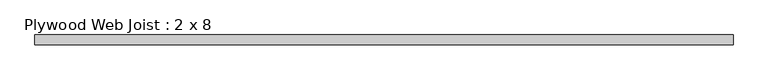
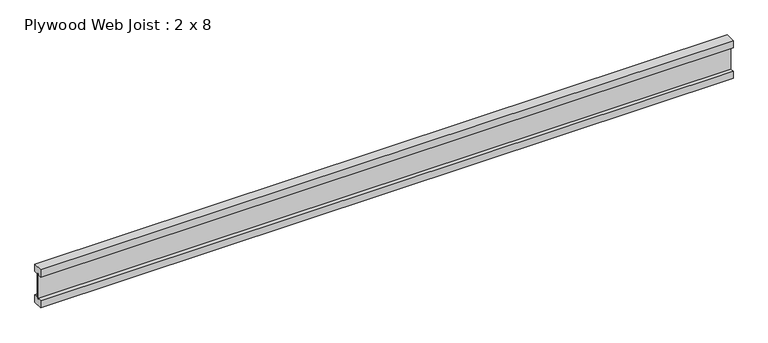
"""IFC4 building model written with IfcOpenShell, lengths in millimetres: beam geometry, Plywood Web Joist : 2 x 8."""

import ifcopenshell
import ifcopenshell.guid

model = None  # the IFC model being written
_history = None  # IfcOwnerHistory: only IFC2X3 demands one
_inside = {}  # id of a spatial element -> (the spatial element, [elements in it])
_under = {}  # id of a project, library or spatial element -> (it, [spatial elements below it])
_declared = {}  # id of a project -> (the project, [libraries it declares])
_typed = {}  # id of a type object -> (the type object, [elements of that type])
_made_of = {}  # id of a material, layer set ... -> (it, [elements and type objects made of it])


def new_model(schema):
    """Start an empty IFC model of exactly this schema.

    Asked for "IFC4X3", IfcOpenShell would pick the latest addendum, in which some entities
    have other attributes; the version numbers below select the first issue.
    IFC2X3 requires an IfcOwnerHistory on every rooted entity: one is made here for all.
    """
    global model, _history
    if schema == "IFC4X3":
        model = ifcopenshell.file(schema_version=(4, 3, 0, 0))
    else:
        model = ifcopenshell.file(schema=schema)
    _inside.clear()
    _under.clear()
    _declared.clear()
    _typed.clear()
    _made_of.clear()
    _history = None
    if model.schema == "IFC2X3":
        org = make("IfcOrganization", Name="unknown")
        user = make(
            "IfcPersonAndOrganization",
            ThePerson=make("IfcPerson", FamilyName="unknown"),
            TheOrganization=org,
        )
        app = make(
            "IfcApplication",
            ApplicationDeveloper=org,
            Version="unknown",
            ApplicationFullName="unknown",
            ApplicationIdentifier="unknown",
        )
        _history = make(
            "IfcOwnerHistory",
            OwningUser=user,
            OwningApplication=app,
            ChangeAction="ADDED",
            CreationDate=0,
        )
    return model


def make(cls, **values):
    """One entity of the class cls with the attributes given. An attribute that is None is left unset."""
    return model.create_entity(
        cls, **{name: value for name, value in values.items() if value is not None}
    )


def rooted(cls, **values):
    """An entity with a GlobalId (a new one), such as an element, a storey or a relation."""
    return make(cls, GlobalId=ifcopenshell.guid.new(), OwnerHistory=_history, **values)


def si_unit(unit_type, name, prefix=None):
    """IfcSIUnit, for example si_unit("LENGTHUNIT", "METRE", prefix="MILLI")."""
    return make("IfcSIUnit", UnitType=unit_type, Prefix=prefix, Name=name)


def assignment(units):
    """IfcUnitAssignment: the units of a project."""
    return None if units is None else make("IfcUnitAssignment", Units=units)


def point(xyz):
    """IfcCartesianPoint."""
    return None if xyz is None else make("IfcCartesianPoint", Coordinates=xyz)


def direction(xyz):
    """IfcDirection."""
    return None if xyz is None else make("IfcDirection", DirectionRatios=xyz)


def frame(location, z_axis=None, x_axis=None):
    """IfcAxis2Placement3D, a coordinate frame: its origin and axes. An axis left out is left unset."""
    return make(
        "IfcAxis2Placement3D",
        Location=point(location),
        Axis=direction(z_axis),
        RefDirection=direction(x_axis),
    )


def origin():
    """The frame at (0, 0, 0) with its axes left unset."""
    return frame((0.0, 0.0, 0.0))


def place(relative_to, where):
    """IfcLocalPlacement: puts the frame where relative to a parent placement (None: the world)."""
    return make(
        "IfcLocalPlacement", PlacementRelTo=relative_to, RelativePlacement=where
    )


def context(
    kind, dimensions, precision=None, world=None, true_north=None, identifier=None
):
    """IfcGeometricRepresentationContext, for example the 3D "Model" context."""
    return make(
        "IfcGeometricRepresentationContext",
        ContextIdentifier=identifier,
        ContextType=kind,
        CoordinateSpaceDimension=dimensions,
        Precision=precision,
        WorldCoordinateSystem=world,
        TrueNorth=true_north,
    )


def project(units=None, contexts=None):
    """IfcProject with its units and contexts."""
    return rooted(
        "IfcProject",
        Name="project",
        RepresentationContexts=contexts,
        UnitsInContext=assignment(units),
    )


def spatial(cls, under=None, at=None, **own):
    """A site, building, storey or space (cls), placed at a placement, below another one or the project."""
    s = rooted(cls, ObjectPlacement=at, **own)
    if under is not None:
        _under.setdefault(under.id(), (under, []))[1].append(s)
    return s


def polyline(points):
    """IfcPolyline through the points."""
    return make("IfcPolyline", Points=[point(p) for p in points])


def outline(outer, holes=None, kind="AREA"):
    """IfcArbitraryClosedProfileDef: a profile drawn as a closed curve; with holes, ...WithVoids."""
    if holes is None:
        return make("IfcArbitraryClosedProfileDef", ProfileType=kind, OuterCurve=outer)
    return make(
        "IfcArbitraryProfileDefWithVoids",
        ProfileType=kind,
        OuterCurve=outer,
        InnerCurves=holes,
    )


def extrude(swept, where, along, depth):
    """IfcExtrudedAreaSolid: the profile swept, set in the frame where, extruded along a direction by depth."""
    return make(
        "IfcExtrudedAreaSolid",
        SweptArea=swept,
        Position=where,
        ExtrudedDirection=direction(along),
        Depth=depth,
    )


def shape(context_of_items, identifier, shape_type, items):
    """IfcShapeRepresentation: the items that make up one representation, for example the "Body"."""
    return make(
        "IfcShapeRepresentation",
        ContextOfItems=context_of_items,
        RepresentationIdentifier=identifier,
        RepresentationType=shape_type,
        Items=items,
    )


def source(mapping_origin, context_of_items, identifier, shape_type, items):
    """IfcRepresentationMap: a shape defined once, which mapped items show again and again."""
    return make(
        "IfcRepresentationMap",
        MappingOrigin=mapping_origin,
        MappedRepresentation=shape(context_of_items, identifier, shape_type, items),
    )


def transform(
    local_origin,
    x_axis=None,
    y_axis=None,
    z_axis=None,
    scale=None,
    scale2=None,
    scale3=None,
    uniform=True,
):
    """IfcCartesianTransformationOperator3D, or its non-uniform kind. x_axis, y_axis, z_axis: its Axis1, 2, 3."""
    if uniform:
        return make(
            "IfcCartesianTransformationOperator3D",
            Axis1=direction(x_axis),
            Axis2=direction(y_axis),
            LocalOrigin=point(local_origin),
            Scale=scale,
            Axis3=direction(z_axis),
        )
    return make(
        "IfcCartesianTransformationOperator3DnonUniform",
        Axis1=direction(x_axis),
        Axis2=direction(y_axis),
        LocalOrigin=point(local_origin),
        Scale=scale,
        Axis3=direction(z_axis),
        Scale2=scale2,
        Scale3=scale3,
    )


def mapped(mapping_source, mapping_target):
    """IfcMappedItem: shows the shape of a source again, moved by a transform."""
    return make(
        "IfcMappedItem", MappingSource=mapping_source, MappingTarget=mapping_target
    )


def made_of(thing, what):
    """Note that an element or type object is made of a material, layer set ...; save() writes the relation."""
    if what is not None:
        _made_of.setdefault(what.id(), (what, []))[1].append(thing)
    return thing


def element(
    cls,
    number,
    at=None,
    inside=None,
    cuts=None,
    type_object=None,
    material=None,
    context=None,
    identifier="Body",
    shape_type=None,
    held_by="IfcProductDefinitionShape",
    body=None,
    shapes=None,
    **own,
):
    """One element of the class cls, such as IfcWall. Its Tag is "e" and its number.

    at: its placement. inside: the storey or other place that contains it. cuts: it is an
    opening in that element (IfcRelVoidsElement). A single representation is given by context,
    identifier, shape_type and body (its items); several are given by shapes. held_by: the class
    of the entity that holds the representations. save() writes the other relations.
    """
    e = rooted(cls, Tag="e%d" % number, ObjectPlacement=at, **own)
    if body is not None:
        shapes = [shape(context, identifier, shape_type, body)]
    if shapes is not None:
        e.Representation = make(held_by, Representations=shapes)
    if inside is not None:
        _inside.setdefault(inside.id(), (inside, []))[1].append(e)
    if cuts is not None:
        rooted(
            "IfcRelVoidsElement", RelatingBuildingElement=cuts, RelatedOpeningElement=e
        )
    if type_object is not None:
        _typed.setdefault(type_object.id(), (type_object, []))[1].append(e)
    return made_of(e, material)


def aggregate(whole, parts):
    """IfcRelAggregates: a whole, such as a stair, and the parts it consists of."""
    return rooted("IfcRelAggregates", RelatingObject=whole, RelatedObjects=parts)


def save(model, path):
    """Write the relations noted so far, then the file.

    IfcRelAggregates (storeys below a building ...), IfcRelContainedInSpatialStructure (elements
    in a storey), IfcRelDefinesByType, IfcRelAssociatesMaterial and IfcRelDeclares: one each for
    every whole, place, type object, material and project.
    """
    for whole, parts in _under.values():
        aggregate(whole, parts)
    for where, things in _inside.values():
        rooted(
            "IfcRelContainedInSpatialStructure",
            RelatedElements=things,
            RelatingStructure=where,
        )
    for kind, things in _typed.values():
        rooted("IfcRelDefinesByType", RelatedObjects=things, RelatingType=kind)
    for what, things in _made_of.values():
        rooted("IfcRelAssociatesMaterial", RelatedObjects=things, RelatingMaterial=what)
    for by, libraries in _declared.values():
        rooted("IfcRelDeclares", RelatingContext=by, RelatedDefinitions=libraries)
    model.write(path)


def plywood_web_joist_2_x_8_8e4157b3(model_context):
    return source(origin(), model_context, "Body", "SweptSolid", [
        extrude(outline(polyline([(-25.4, 101.6), (25.4, 101.6), (25.4, 63.5), (4.7625, 63.5), (4.7625, 69.85), (-4.7625, 69.85), (-4.7625, 63.5), (-25.4, 63.5), (-25.4, 101.6)])), frame((-1758.95, 0.0, 0.0), z_axis=(1.0, 0.0, 0.0), x_axis=(0.0, 1.0, 0.0)), (0.0, 0.0, 1.0), 3517.9),
        extrude(outline(polyline([(25.4, -63.5), (25.4, -101.6), (-25.4, -101.6), (-25.4, -63.5), (-4.7625, -63.5), (-4.7625, -69.1160374), (4.7625, -69.1160374), (4.7625, -63.5), (25.4, -63.5)])), frame((-1758.95, 0.0, 0.0), z_axis=(1.0, 0.0, 0.0), x_axis=(0.0, 1.0, 0.0)), (0.0, 0.0, 1.0), 3517.9),
        extrude(outline(polyline([(1758.95, 4.7625), (1758.95, -4.7625), (-1758.95, -4.7625), (-1758.95, 4.7625), (1758.95, 4.7625)])), frame((0.0, 0.0, -69.1160374), z_axis=(0.0, 0.0, 1.0), x_axis=(1.0, 0.0, 0.0)), (0.0, 0.0, 1.0), 138.9660374),
    ])


if __name__ == "__main__":
    model = new_model("IFC4")
    model_context = context("Model", 3, world=origin())
    ifc_project = project(units=[si_unit("LENGTHUNIT", "METRE", prefix="MILLI")], contexts=[model_context])
    site = spatial("IfcSite", under=ifc_project)
    building = spatial("IfcBuilding", under=site)
    placement = place(None, origin())
    plywood_web_joist_2_x_8_shape = plywood_web_joist_2_x_8_8e4157b3(model_context)
    element("IfcBeam", 1, ObjectType="Plywood Web Joist : 2 x 8", at=placement, inside=building, context=model_context, shape_type="MappedRepresentation", body=[
        mapped(plywood_web_joist_2_x_8_shape, transform((0.0, 0.0, 0.0), x_axis=(1.0, 0.0, 0.0), y_axis=(0.0, 1.0, 0.0), z_axis=(0.0, 0.0, 1.0))),
    ])
    save(model, "model.ifc")

# Revit data of these elements
# Type "Plywood Web Joist : 2 x 8"
#   Assembly Code = "B10"
#   Length [instance default] = 5' - 0"
#   b = 0' - 2"
#   d = 0' - 8"
#   Structural Material [instance default] = Softwood, Lumber
# Element 1 (IfcBeam, "Plywood Web Joist : 2 x 8")
#   Materials on its faces: "Softwood, Lumber"
# Materials
#   "Softwood, Lumber": class "Wood", colour RGB 144 113 62, transparency 0, Description = "Pinus Echinata", Cost = 0
